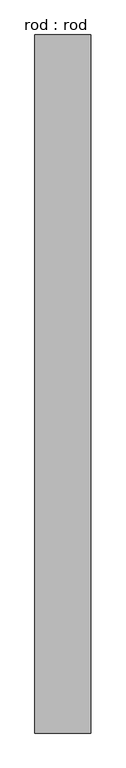
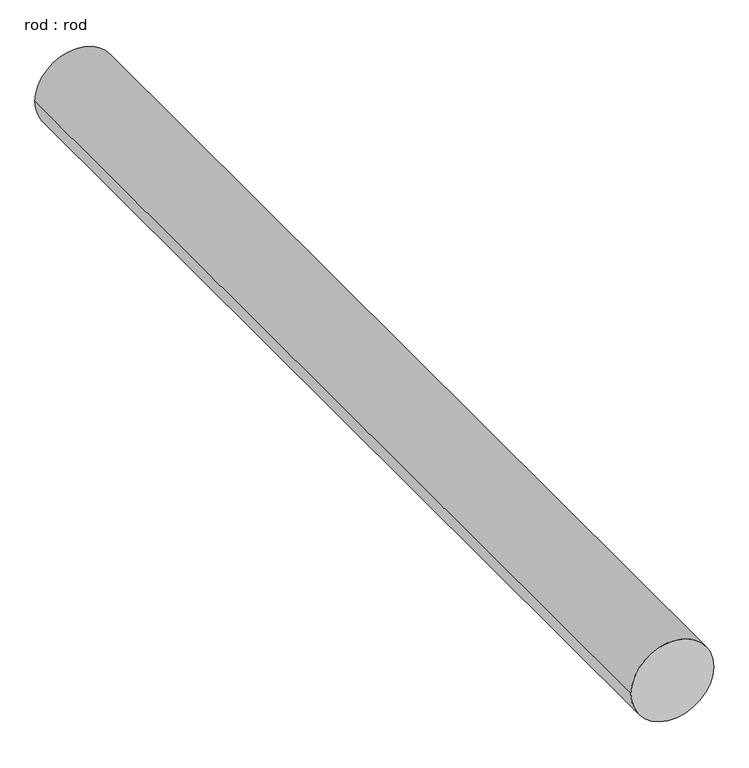
"""IFC4 building model written with IfcOpenShell, lengths in millimetres: proxy geometry, rod : rod."""

from ifc_helpers import new_model, si_unit, point, frame, frame_2d, origin, place, context, project, spatial, circle_curve, trimmed, segment, composite_curve, outline, extrude, source, transform, mapped, element, save


def rod_rod_b2d37f7d(model_context):
    return source(origin(), model_context, "Body", "SweptSolid", [
        extrude(outline(composite_curve([segment(trimmed(circle_curve(frame_2d((0.0108462, 0.0)), 200.0), [point((0.0108462, 200.0))], [point((0.0108462, -200.0))], False, "CARTESIAN"), True, "CONTINUOUS"), segment(trimmed(circle_curve(frame_2d((0.0108462, 0.0)), 200.0), [point((0.0108462, -200.0))], [point((0.0108462, 200.0))], False, "CARTESIAN"), True, "CONTINUOUS")], self_intersect=False)), frame((0.0, 1592.7286153, 0.0), z_axis=(0.0, 1.0, 0.0), x_axis=(0.0, 0.0, 1.0)), (0.0, 0.0, 1.0), 5000.0),
    ])


if __name__ == "__main__":
    model = new_model("IFC4")
    model_context = context("Model", 3, world=origin())
    ifc_project = project(units=[si_unit("LENGTHUNIT", "METRE", prefix="MILLI")], contexts=[model_context])
    site = spatial("IfcSite", under=ifc_project)
    building = spatial("IfcBuilding", under=site)
    placement = place(None, origin())
    rod_rod_shape = rod_rod_b2d37f7d(model_context)
    element("IfcBuildingElementProxy", 1, Name="rod : rod", ObjectType="rod : rod", at=placement, inside=building, context=model_context, shape_type="MappedRepresentation", body=[
        mapped(rod_rod_shape, transform((0.0, 0.0, 0.0), x_axis=(1.0, 0.0, 0.0), y_axis=(0.0, 1.0, 0.0), z_axis=(0.0, 0.0, 1.0))),
    ])
    save(model, "model.ifc")

# Revit data of these elements
# Type "rod : rod"
#   Default Elevation = 0
